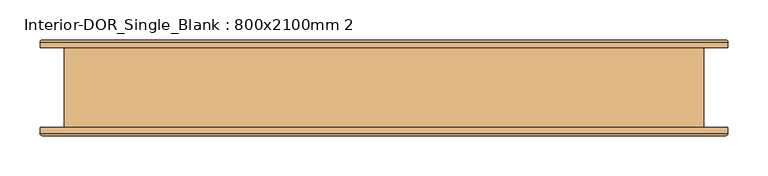
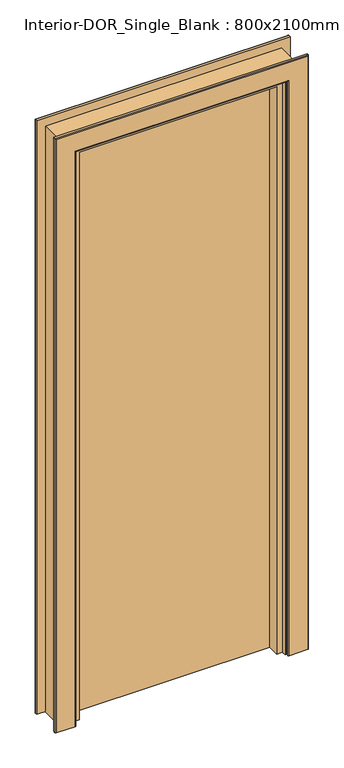
"""IFC4 building model written with IfcOpenShell, lengths in millimetres: door geometry, Interior-DOR_Single_Blank : 800x2100mm 2."""

import ifcopenshell
import ifcopenshell.guid

model = None  # the IFC model being written
_history = None  # IfcOwnerHistory: only IFC2X3 demands one
_inside = {}  # id of a spatial element -> (the spatial element, [elements in it])
_under = {}  # id of a project, library or spatial element -> (it, [spatial elements below it])
_declared = {}  # id of a project -> (the project, [libraries it declares])
_typed = {}  # id of a type object -> (the type object, [elements of that type])
_made_of = {}  # id of a material, layer set ... -> (it, [elements and type objects made of it])


def new_model(schema):
    """Start an empty IFC model of exactly this schema.

    Asked for "IFC4X3", IfcOpenShell would pick the latest addendum, in which some entities
    have other attributes; the version numbers below select the first issue.
    IFC2X3 requires an IfcOwnerHistory on every rooted entity: one is made here for all.
    """
    global model, _history
    if schema == "IFC4X3":
        model = ifcopenshell.file(schema_version=(4, 3, 0, 0))
    else:
        model = ifcopenshell.file(schema=schema)
    _inside.clear()
    _under.clear()
    _declared.clear()
    _typed.clear()
    _made_of.clear()
    _history = None
    if model.schema == "IFC2X3":
        org = make("IfcOrganization", Name="unknown")
        user = make(
            "IfcPersonAndOrganization",
            ThePerson=make("IfcPerson", FamilyName="unknown"),
            TheOrganization=org,
        )
        app = make(
            "IfcApplication",
            ApplicationDeveloper=org,
            Version="unknown",
            ApplicationFullName="unknown",
            ApplicationIdentifier="unknown",
        )
        _history = make(
            "IfcOwnerHistory",
            OwningUser=user,
            OwningApplication=app,
            ChangeAction="ADDED",
            CreationDate=0,
        )
    return model


def make(cls, **values):
    """One entity of the class cls with the attributes given. An attribute that is None is left unset."""
    return model.create_entity(
        cls, **{name: value for name, value in values.items() if value is not None}
    )


def rooted(cls, **values):
    """An entity with a GlobalId (a new one), such as an element, a storey or a relation."""
    return make(cls, GlobalId=ifcopenshell.guid.new(), OwnerHistory=_history, **values)


def si_unit(unit_type, name, prefix=None):
    """IfcSIUnit, for example si_unit("LENGTHUNIT", "METRE", prefix="MILLI")."""
    return make("IfcSIUnit", UnitType=unit_type, Prefix=prefix, Name=name)


def assignment(units):
    """IfcUnitAssignment: the units of a project."""
    return None if units is None else make("IfcUnitAssignment", Units=units)


def point(xyz):
    """IfcCartesianPoint."""
    return None if xyz is None else make("IfcCartesianPoint", Coordinates=xyz)


def direction(xyz):
    """IfcDirection."""
    return None if xyz is None else make("IfcDirection", DirectionRatios=xyz)


def frame(location, z_axis=None, x_axis=None):
    """IfcAxis2Placement3D, a coordinate frame: its origin and axes. An axis left out is left unset."""
    return make(
        "IfcAxis2Placement3D",
        Location=point(location),
        Axis=direction(z_axis),
        RefDirection=direction(x_axis),
    )


def origin():
    """The frame at (0, 0, 0) with its axes left unset."""
    return frame((0.0, 0.0, 0.0))


def origin_with_axes():
    """The frame at (0, 0, 0) with the z axis (0, 0, 1) and the x axis (1, 0, 0) written out."""
    return frame((0.0, 0.0, 0.0), z_axis=(0.0, 0.0, 1.0), x_axis=(1.0, 0.0, 0.0))


def place(relative_to, where):
    """IfcLocalPlacement: puts the frame where relative to a parent placement (None: the world)."""
    return make(
        "IfcLocalPlacement", PlacementRelTo=relative_to, RelativePlacement=where
    )


def context(
    kind, dimensions, precision=None, world=None, true_north=None, identifier=None
):
    """IfcGeometricRepresentationContext, for example the 3D "Model" context."""
    return make(
        "IfcGeometricRepresentationContext",
        ContextIdentifier=identifier,
        ContextType=kind,
        CoordinateSpaceDimension=dimensions,
        Precision=precision,
        WorldCoordinateSystem=world,
        TrueNorth=true_north,
    )


def project(units=None, contexts=None):
    """IfcProject with its units and contexts."""
    return rooted(
        "IfcProject",
        Name="project",
        RepresentationContexts=contexts,
        UnitsInContext=assignment(units),
    )


def spatial(cls, under=None, at=None, **own):
    """A site, building, storey or space (cls), placed at a placement, below another one or the project."""
    s = rooted(cls, ObjectPlacement=at, **own)
    if under is not None:
        _under.setdefault(under.id(), (under, []))[1].append(s)
    return s


def polyline(points):
    """IfcPolyline through the points."""
    return make("IfcPolyline", Points=[point(p) for p in points])


def circle_curve(where, radius):
    """IfcCircle in the frame where."""
    return make("IfcCircle", Position=where, Radius=radius)


def ellipse_curve(where, semi_axis1, semi_axis2):
    """IfcEllipse in the frame where."""
    return make(
        "IfcEllipse", Position=where, SemiAxis1=semi_axis1, SemiAxis2=semi_axis2
    )


def outline(outer, holes=None, kind="AREA"):
    """IfcArbitraryClosedProfileDef: a profile drawn as a closed curve; with holes, ...WithVoids."""
    if holes is None:
        return make("IfcArbitraryClosedProfileDef", ProfileType=kind, OuterCurve=outer)
    return make(
        "IfcArbitraryProfileDefWithVoids",
        ProfileType=kind,
        OuterCurve=outer,
        InnerCurves=holes,
    )


def extrude(swept, where, along, depth):
    """IfcExtrudedAreaSolid: the profile swept, set in the frame where, extruded along a direction by depth."""
    return make(
        "IfcExtrudedAreaSolid",
        SweptArea=swept,
        Position=where,
        ExtrudedDirection=direction(along),
        Depth=depth,
    )


def faces_of(points, faces, orient=None, outer=None):
    """IfcFace entities. A face is a list of loops; a loop is a list of indices into points, from 0.

    orient and outer hold one flag for each loop. By default every Orientation is true, the
    first loop of a face is its IfcFaceOuterBound and the others are IfcFaceBound.
    """
    made = []
    for i, loops in enumerate(faces):
        bounds = []
        for j, loop in enumerate(loops):
            is_outer = j == 0 if outer is None else outer[i][j]
            bounds.append(
                make(
                    "IfcFaceOuterBound" if is_outer else "IfcFaceBound",
                    Bound=make("IfcPolyLoop", Polygon=[points[k] for k in loop]),
                    Orientation=True if orient is None else orient[i][j],
                )
            )
        made.append(make("IfcFace", Bounds=bounds))
    return made


def faceted_brep(points, faces, orient=None, outer=None, voids=None):
    """IfcFacetedBrep: a solid bounded by flat faces; with voids (closed shells), ...WithVoids."""
    shared = [point(p) for p in points]
    hull = make("IfcClosedShell", CfsFaces=faces_of(shared, faces, orient, outer))
    if voids is None:
        return make("IfcFacetedBrep", Outer=hull)
    return make(
        "IfcFacetedBrepWithVoids",
        Outer=hull,
        Voids=[
            make(cls, CfsFaces=faces_of(shared, fs, o, b)) for cls, fs, o, b in voids
        ],
    )


def shape(context_of_items, identifier, shape_type, items):
    """IfcShapeRepresentation: the items that make up one representation, for example the "Body"."""
    return make(
        "IfcShapeRepresentation",
        ContextOfItems=context_of_items,
        RepresentationIdentifier=identifier,
        RepresentationType=shape_type,
        Items=items,
    )


def source(mapping_origin, context_of_items, identifier, shape_type, items):
    """IfcRepresentationMap: a shape defined once, which mapped items show again and again."""
    return make(
        "IfcRepresentationMap",
        MappingOrigin=mapping_origin,
        MappedRepresentation=shape(context_of_items, identifier, shape_type, items),
    )


def transform(
    local_origin,
    x_axis=None,
    y_axis=None,
    z_axis=None,
    scale=None,
    scale2=None,
    scale3=None,
    uniform=True,
):
    """IfcCartesianTransformationOperator3D, or its non-uniform kind. x_axis, y_axis, z_axis: its Axis1, 2, 3."""
    if uniform:
        return make(
            "IfcCartesianTransformationOperator3D",
            Axis1=direction(x_axis),
            Axis2=direction(y_axis),
            LocalOrigin=point(local_origin),
            Scale=scale,
            Axis3=direction(z_axis),
        )
    return make(
        "IfcCartesianTransformationOperator3DnonUniform",
        Axis1=direction(x_axis),
        Axis2=direction(y_axis),
        LocalOrigin=point(local_origin),
        Scale=scale,
        Axis3=direction(z_axis),
        Scale2=scale2,
        Scale3=scale3,
    )


def mapped(mapping_source, mapping_target):
    """IfcMappedItem: shows the shape of a source again, moved by a transform."""
    return make(
        "IfcMappedItem", MappingSource=mapping_source, MappingTarget=mapping_target
    )


def made_of(thing, what):
    """Note that an element or type object is made of a material, layer set ...; save() writes the relation."""
    if what is not None:
        _made_of.setdefault(what.id(), (what, []))[1].append(thing)
    return thing


def element(
    cls,
    number,
    at=None,
    inside=None,
    cuts=None,
    type_object=None,
    material=None,
    context=None,
    identifier="Body",
    shape_type=None,
    held_by="IfcProductDefinitionShape",
    body=None,
    shapes=None,
    **own,
):
    """One element of the class cls, such as IfcWall. Its Tag is "e" and its number.

    at: its placement. inside: the storey or other place that contains it. cuts: it is an
    opening in that element (IfcRelVoidsElement). A single representation is given by context,
    identifier, shape_type and body (its items); several are given by shapes. held_by: the class
    of the entity that holds the representations. save() writes the other relations.
    """
    e = rooted(cls, Tag="e%d" % number, ObjectPlacement=at, **own)
    if body is not None:
        shapes = [shape(context, identifier, shape_type, body)]
    if shapes is not None:
        e.Representation = make(held_by, Representations=shapes)
    if inside is not None:
        _inside.setdefault(inside.id(), (inside, []))[1].append(e)
    if cuts is not None:
        rooted(
            "IfcRelVoidsElement", RelatingBuildingElement=cuts, RelatedOpeningElement=e
        )
    if type_object is not None:
        _typed.setdefault(type_object.id(), (type_object, []))[1].append(e)
    return made_of(e, material)


def aggregate(whole, parts):
    """IfcRelAggregates: a whole, such as a stair, and the parts it consists of."""
    return rooted("IfcRelAggregates", RelatingObject=whole, RelatedObjects=parts)


def save(model, path):
    """Write the relations noted so far, then the file.

    IfcRelAggregates (storeys below a building ...), IfcRelContainedInSpatialStructure (elements
    in a storey), IfcRelDefinesByType, IfcRelAssociatesMaterial and IfcRelDeclares: one each for
    every whole, place, type object, material and project.
    """
    for whole, parts in _under.values():
        aggregate(whole, parts)
    for where, things in _inside.values():
        rooted(
            "IfcRelContainedInSpatialStructure",
            RelatedElements=things,
            RelatingStructure=where,
        )
    for kind, things in _typed.values():
        rooted("IfcRelDefinesByType", RelatedObjects=things, RelatingType=kind)
    for what, things in _made_of.values():
        rooted("IfcRelAssociatesMaterial", RelatedObjects=things, RelatingMaterial=what)
    for by, libraries in _declared.values():
        rooted("IfcRelDeclares", RelatingContext=by, RelatedDefinitions=libraries)
    model.write(path)


def plane_surface(at):
    """IfcPlane: the flat surface through the origin of the frame at, square to its z axis."""
    return make("IfcPlane", Position=at)


def cylinder_surface(at, radius):
    """IfcCylindricalSurface: all points at the distance radius from the z axis of the frame at."""
    return make("IfcCylindricalSurface", Position=at, Radius=radius)


def advanced_brep(points, edges, surfaces, faces):
    """IfcAdvancedBrep: a solid bounded by faces that lie on surfaces and meet in shared edges.

    An edge is (start, end): straight between two places in points (the first is 0);
    or (start, end, curve); or (start, end, curve, False) where it runs against its curve.
    A face is (place in surfaces, loops), or (place, loops, False) where it looks against
    its surface's normal. A loop lists edges by number (the first is 1), with a minus sign
    where the edge is run from its end to its start. The first loop is the outer one.
    """
    corners = [point(p) for p in points]
    vertices = [make("IfcVertexPoint", VertexGeometry=c) for c in corners]
    made = []
    for start, end, *more in edges:
        made.append(
            make(
                "IfcEdgeCurve",
                EdgeStart=vertices[start],
                EdgeEnd=vertices[end],
                EdgeGeometry=more[0] if more else make("IfcPolyline", Points=[corners[start], corners[end]]),
                SameSense=more[1] if len(more) > 1 else True,
            )
        )
    hull = []
    for where, loops, *sense in faces:
        bounds = []
        for j, loop in enumerate(loops):
            ring = [make("IfcOrientedEdge", EdgeElement=made[abs(k) - 1], Orientation=k > 0) for k in loop]
            bounds.append(
                make(
                    "IfcFaceOuterBound" if j == 0 else "IfcFaceBound",
                    Bound=make("IfcEdgeLoop", EdgeList=ring),
                    Orientation=True,
                )
            )
        hull.append(make("IfcAdvancedFace", Bounds=bounds, FaceSurface=surfaces[where], SameSense=sense[0] if sense else True))
    return make("IfcAdvancedBrep", Outer=make("IfcClosedShell", CfsFaces=hull))


def interior_dor_single_blank_800x2100mm_2_9dcdbc73(model_context):
    return source(origin(), model_context, "Body", "SolidModel", [
        advanced_brep(
        [(-360.0, 50.0, 0.0), (-430.0, 50.0, 0.0), (-430.0, 57.0, 0.0), (-427.0, 60.0, 0.0), (-363.0, 60.0, 0.0), (-360.0, 57.0, 0.0), (-360.0, 57.0, 2060.0), (-360.0, 50.0, 2060.0), (-363.0, 60.0, 2063.0), (-427.0, 60.0, 2127.0), (427.0, 60.0, 2127.0), (427.0, 60.0, 0.0), (363.0, 60.0, 0.0), (363.0, 60.0, 2063.0), (-430.0, 57.0, 2130.0), (-430.0, 50.0, 2130.0), (360.0, 50.0, 2060.0), (360.0, 50.0, 0.0), (430.0, 50.0, 0.0), (430.0, 50.0, 2130.0), (360.0, 57.0, 0.0), (360.0, 57.0, 2060.0), (430.0, 57.0, 0.0), (430.0, 57.0, 2130.0)],
        [
            (0, 1),
            (1, 2),
            (2, 3, circle_curve(frame((-427.0, 57.0, 0.0), z_axis=(0.0, 0.0, -1.0), x_axis=(-1.0, 0.0, 0.0)), 3.0)),
            (3, 4),
            (4, 5, circle_curve(frame((-363.0, 57.0, 0.0), z_axis=(0.0, 0.0, -1.0), x_axis=(-1.0, 0.0, 0.0)), 3.0)),
            (5, 0),
            (5, 6),
            (6, 7),
            (7, 0),
            (4, 8),
            (8, 6, ellipse_curve(frame((-363.0, 57.0, 2063.0), z_axis=(-0.7071067811865475, 0.0, -0.7071067811865475), x_axis=(0.7071067811865474, 0.0, -0.7071067811865476)), 4.2426407, 3.0)),
            (3, 9),
            (9, 10),
            (10, 11),
            (11, 12),
            (12, 13),
            (13, 8),
            (2, 14),
            (14, 9, ellipse_curve(frame((-427.0, 57.0, 2127.0), z_axis=(-0.7071067811865475, 0.0, -0.7071067811865475), x_axis=(0.7071067811865474, 0.0, -0.7071067811865476)), 4.2426407, 3.0)),
            (1, 15),
            (15, 14),
            (7, 16),
            (16, 17),
            (17, 18),
            (18, 19),
            (19, 15),
            (12, 20, circle_curve(frame((363.0, 57.0, 0.0), z_axis=(0.0, 0.0, 1.0), x_axis=(1.0, 0.0, 0.0)), 3.0)),
            (20, 21),
            (21, 13, ellipse_curve(frame((363.0, 57.0, 2063.0), z_axis=(0.7071067811865475, 0.0, -0.7071067811865475), x_axis=(0.7071067811865474, 0.0, 0.7071067811865476)), 4.2426407, 3.0)),
            (17, 20),
            (11, 22, circle_curve(frame((427.0, 57.0, 0.0), z_axis=(0.0, 0.0, -1.0), x_axis=(1.0, 0.0, 0.0)), 3.0)),
            (22, 18),
            (23, 22),
            (10, 23, ellipse_curve(frame((427.0, 57.0, 2127.0), z_axis=(0.7071067811865475, 0.0, -0.7071067811865475), x_axis=(0.7071067811865474, 0.0, 0.7071067811865476)), 4.2426407, 3.0)),
            (23, 19),
            (16, 21),
            (6, 21),
            (14, 23),
        ],
        [
            plane_surface(frame((-400.0, -50.0, 0.0), z_axis=(0.0, 0.0, -1.0), x_axis=(0.0, 1.0, 0.0))),
            plane_surface(frame((-360.0, 50.0, 0.0), z_axis=(1.0, 0.0, 0.0), x_axis=(0.0, 0.0, 1.0))),
            cylinder_surface(frame((-363.0, 57.0, 0.0), z_axis=(0.0, 0.0, -1.0), x_axis=(-1.0, 0.0, 0.0)), 3.0),
            plane_surface(frame((-363.0, 60.0, 0.0), z_axis=(0.0, 1.0, 0.0), x_axis=(0.0, 0.0, 1.0))),
            cylinder_surface(frame((-427.0, 57.0, 0.0), z_axis=(0.0, 0.0, -1.0), x_axis=(-1.0, 0.0, 0.0)), 3.0),
            plane_surface(frame((-430.0, 57.0, 0.0), z_axis=(-1.0, 0.0, 0.0), x_axis=(0.0, 0.0, 1.0))),
            plane_surface(frame((-430.0, 50.0, 0.0), z_axis=(0.0, -1.0, 0.0), x_axis=(0.0, 0.0, 1.0))),
            cylinder_surface(frame((363.0, 57.0, 2100.0), z_axis=(0.0, 0.0, 1.0), x_axis=(1.0, 0.0, 0.0)), 3.0),
            plane_surface(frame((400.0, -50.0, 0.0), z_axis=(0.0, 0.0, -1.0), x_axis=(0.0, 1.0, 0.0))),
            cylinder_surface(frame((427.0, 57.0, 2100.0), z_axis=(0.0, 0.0, 1.0), x_axis=(1.0, 0.0, 0.0)), 3.0),
            plane_surface(frame((430.0, 57.0, 2130.0), z_axis=(1.0, 0.0, 0.0), x_axis=(0.0, 0.0, -1.0))),
            plane_surface(frame((360.0, 50.0, 2060.0), z_axis=(-1.0, 0.0, 0.0), x_axis=(0.0, 0.0, -1.0))),
            plane_surface(frame((-360.0, 50.0, 2060.0), z_axis=(0.0, 0.0, -1.0), x_axis=(1.0, 0.0, 0.0))),
            cylinder_surface(frame((-400.0, 57.0, 2063.0), z_axis=(-1.0, 0.0, 0.0), x_axis=(0.0, 0.0, 1.0)), 3.0),
            cylinder_surface(frame((-400.0, 57.0, 2127.0), z_axis=(-1.0, 0.0, 0.0), x_axis=(0.0, 0.0, 1.0)), 3.0),
            plane_surface(frame((-430.0, 57.0, 2130.0), z_axis=(0.0, 0.0, 1.0), x_axis=(1.0, 0.0, 0.0))),
        ],
        [
            (0, [[1, 2, 3, 4, 5, 6]]),
            (1, [[7, 8, 9, -6]]),
            (2, [[10, 11, -7, -5]]),
            (3, [[12, 13, 14, 15, 16, 17, -10, -4]]),
            (4, [[18, 19, -12, -3]]),
            (5, [[20, 21, -18, -2]]),
            (6, [[-9, 22, 23, 24, 25, 26, -20, -1]]),
            (7, [[-16, 27, 28, 29]]),
            (8, [[30, -27, -15, 31, 32, -24]]),
            (9, [[33, -31, -14, 34]]),
            (10, [[-25, -32, -33, 35]]),
            (11, [[-28, -30, -23, 36]]),
            (12, [[37, -36, -22, -8]]),
            (13, [[-17, -29, -37, -11]]),
            (14, [[38, -34, -13, -19]]),
            (15, [[-26, -35, -38, -21]]),
        ],
    ),
        advanced_brep(
        [(-430.0, -50.0, 0.0), (-360.0, -50.0, 0.0), (-360.0, -57.0, 0.0), (-363.0, -60.0, 0.0), (-427.0, -60.0, 0.0), (-430.0, -57.0, 0.0), (-430.0, -57.0, 2130.0), (-430.0, -50.0, 2130.0), (-427.0, -60.0, 2127.0), (-363.0, -60.0, 2063.0), (363.0, -60.0, 2063.0), (363.0, -60.0, 0.0), (427.0, -60.0, 0.0), (427.0, -60.0, 2127.0), (-360.0, -57.0, 2060.0), (-360.0, -50.0, 2060.0), (430.0, -50.0, 2130.0), (430.0, -50.0, 0.0), (360.0, -50.0, 0.0), (360.0, -50.0, 2060.0), (430.0, -57.0, 0.0), (430.0, -57.0, 2130.0), (360.0, -57.0, 0.0), (360.0, -57.0, 2060.0)],
        [
            (0, 1),
            (1, 2),
            (2, 3, circle_curve(frame((-363.0, -57.0, 0.0), z_axis=(0.0, 0.0, -1.0), x_axis=(-1.0, 0.0, 0.0)), 3.0)),
            (3, 4),
            (4, 5, circle_curve(frame((-427.0, -57.0, 0.0), z_axis=(0.0, 0.0, -1.0), x_axis=(-1.0, 0.0, 0.0)), 3.0)),
            (5, 0),
            (5, 6),
            (6, 7),
            (7, 0),
            (4, 8),
            (8, 6, ellipse_curve(frame((-427.0, -57.0, 2127.0), z_axis=(-0.7071067811865475, 0.0, -0.7071067811865475), x_axis=(0.7071067811865474, 0.0, -0.7071067811865476)), 4.2426407, 3.0)),
            (3, 9),
            (9, 10),
            (10, 11),
            (11, 12),
            (12, 13),
            (13, 8),
            (2, 14),
            (14, 9, ellipse_curve(frame((-363.0, -57.0, 2063.0), z_axis=(-0.7071067811865475, 0.0, -0.7071067811865475), x_axis=(0.7071067811865474, 0.0, -0.7071067811865476)), 4.2426407, 3.0)),
            (1, 15),
            (15, 14),
            (7, 16),
            (16, 17),
            (17, 18),
            (18, 19),
            (19, 15),
            (12, 20, circle_curve(frame((427.0, -57.0, 0.0), z_axis=(0.0, 0.0, 1.0), x_axis=(1.0, 0.0, 0.0)), 3.0)),
            (20, 21),
            (21, 13, ellipse_curve(frame((427.0, -57.0, 2127.0), z_axis=(0.7071067811865475, 0.0, -0.7071067811865475), x_axis=(0.7071067811865474, 0.0, 0.7071067811865476)), 4.2426407, 3.0)),
            (17, 20),
            (11, 22, circle_curve(frame((363.0, -57.0, 0.0), z_axis=(0.0, 0.0, -1.0), x_axis=(1.0, 0.0, 0.0)), 3.0)),
            (22, 18),
            (23, 22),
            (10, 23, ellipse_curve(frame((363.0, -57.0, 2063.0), z_axis=(0.7071067811865475, 0.0, -0.7071067811865475), x_axis=(0.7071067811865474, 0.0, 0.7071067811865476)), 4.2426407, 3.0)),
            (23, 19),
            (16, 21),
            (6, 21),
            (14, 23),
        ],
        [
            plane_surface(frame((-400.0, -50.0, 0.0), z_axis=(0.0, 0.0, -1.0), x_axis=(0.0, 1.0, 0.0))),
            plane_surface(frame((-430.0, -50.0, 0.0), z_axis=(-1.0, 0.0, 0.0), x_axis=(0.0, 0.0, 1.0))),
            cylinder_surface(frame((-427.0, -57.0, 0.0), z_axis=(0.0, 0.0, -1.0), x_axis=(-1.0, 0.0, 0.0)), 3.0),
            plane_surface(frame((-427.0, -60.0, 0.0), z_axis=(0.0, -1.0, 0.0), x_axis=(0.0, 0.0, 1.0))),
            cylinder_surface(frame((-363.0, -57.0, 0.0), z_axis=(0.0, 0.0, -1.0), x_axis=(-1.0, 0.0, 0.0)), 3.0),
            plane_surface(frame((-360.0, -57.0, 0.0), z_axis=(1.0, 0.0, 0.0), x_axis=(0.0, 0.0, 1.0))),
            plane_surface(frame((-360.0, -50.0, 0.0), z_axis=(0.0, 1.0, 0.0), x_axis=(0.0, 0.0, 1.0))),
            cylinder_surface(frame((427.0, -57.0, 2100.0), z_axis=(0.0, 0.0, 1.0), x_axis=(1.0, 0.0, 0.0)), 3.0),
            plane_surface(frame((400.0, -50.0, 0.0), z_axis=(0.0, 0.0, -1.0), x_axis=(0.0, 1.0, 0.0))),
            cylinder_surface(frame((363.0, -57.0, 2100.0), z_axis=(0.0, 0.0, 1.0), x_axis=(1.0, 0.0, 0.0)), 3.0),
            plane_surface(frame((360.0, -57.0, 2060.0), z_axis=(-1.0, 0.0, 0.0), x_axis=(0.0, 0.0, -1.0))),
            plane_surface(frame((430.0, -50.0, 2130.0), z_axis=(1.0, 0.0, 0.0), x_axis=(0.0, 0.0, -1.0))),
            plane_surface(frame((-430.0, -50.0, 2130.0), z_axis=(0.0, 0.0, 1.0), x_axis=(1.0, 0.0, 0.0))),
            cylinder_surface(frame((-400.0, -57.0, 2127.0), z_axis=(-1.0, 0.0, 0.0), x_axis=(0.0, 0.0, 1.0)), 3.0),
            cylinder_surface(frame((-400.0, -57.0, 2063.0), z_axis=(-1.0, 0.0, 0.0), x_axis=(0.0, 0.0, 1.0)), 3.0),
            plane_surface(frame((-360.0, -57.0, 2060.0), z_axis=(0.0, 0.0, -1.0), x_axis=(1.0, 0.0, 0.0))),
        ],
        [
            (0, [[1, 2, 3, 4, 5, 6]]),
            (1, [[7, 8, 9, -6]]),
            (2, [[10, 11, -7, -5]]),
            (3, [[12, 13, 14, 15, 16, 17, -10, -4]]),
            (4, [[18, 19, -12, -3]]),
            (5, [[20, 21, -18, -2]]),
            (6, [[-9, 22, 23, 24, 25, 26, -20, -1]]),
            (7, [[-16, 27, 28, 29]]),
            (8, [[30, -27, -15, 31, 32, -24]]),
            (9, [[33, -31, -14, 34]]),
            (10, [[-25, -32, -33, 35]]),
            (11, [[-28, -30, -23, 36]]),
            (12, [[37, -36, -22, -8]]),
            (13, [[-17, -29, -37, -11]]),
            (14, [[38, -34, -13, -19]]),
            (15, [[-26, -35, -38, -21]]),
        ],
    ),
        faceted_brep([(-400.0, -50.0, 0.0), (-400.0, 50.0, 0.0), (-355.0, 50.0, 0.0), (-355.0, 5.0, 0.0), (-335.0, 5.0, 0.0), (-335.0, -35.0, 0.0), (-355.0, -35.0, 0.0), (-355.0, -50.0, 0.0), (-355.0, -50.0, 2055.0), (355.0, -50.0, 2055.0), (355.0, -50.0, 0.0), (400.0, -50.0, 0.0), (400.0, -50.0, 2100.0), (-400.0, -50.0, 2100.0), (-355.0, -35.0, 2055.0), (-335.0, -35.0, 2035.0), (335.0, -35.0, 2035.0), (335.0, -35.0, 0.0), (355.0, -35.0, 0.0), (355.0, -35.0, 2055.0), (-335.0, 5.0, 2035.0), (-355.0, 5.0, 2055.0), (355.0, 5.0, 2055.0), (355.0, 5.0, 0.0), (335.0, 5.0, 0.0), (335.0, 5.0, 2035.0), (-355.0, 50.0, 2055.0), (-400.0, 50.0, 2100.0), (400.0, 50.0, 2100.0), (400.0, 50.0, 0.0), (355.0, 50.0, 0.0), (355.0, 50.0, 2055.0)], [[[0, 1, 2, 3, 4, 5, 6, 7]], [[7, 8, 9, 10, 11, 12, 13, 0]], [[6, 14, 8, 7]], [[5, 15, 16, 17, 18, 19, 14, 6]], [[4, 20, 15, 5]], [[3, 21, 22, 23, 24, 25, 20, 4]], [[2, 26, 21, 3]], [[1, 27, 28, 29, 30, 31, 26, 2]], [[0, 13, 27, 1]], [[12, 11, 29, 28]], [[11, 10, 18, 17, 24, 23, 30, 29]], [[19, 18, 10, 9]], [[25, 24, 17, 16]], [[31, 30, 23, 22]], [[20, 25, 16, 15]], [[26, 31, 22, 21]], [[13, 12, 28, 27]], [[14, 19, 9, 8]]]),
        extrude(outline(polyline([(355.0, 50.0), (355.0, 5.0), (-355.0, 5.0), (-355.0, 50.0), (355.0, 50.0)])), origin_with_axes(), (0.0, 0.0, 1.0), 2055.0),
    ])


if __name__ == "__main__":
    model = new_model("IFC4")
    model_context = context("Model", 3, world=origin())
    ifc_project = project(units=[si_unit("LENGTHUNIT", "METRE", prefix="MILLI")], contexts=[model_context])
    site = spatial("IfcSite", under=ifc_project)
    building = spatial("IfcBuilding", under=site)
    placement = place(None, origin())
    interior_dor_single_blank_800x2100mm_2_shape = interior_dor_single_blank_800x2100mm_2_9dcdbc73(model_context)
    element("IfcDoor", 1, ObjectType="Interior-DOR_Single_Blank : 800x2100mm 2", at=placement, inside=building, context=model_context, shape_type="MappedRepresentation", body=[
        mapped(interior_dor_single_blank_800x2100mm_2_shape, transform((0.0, 0.0, 0.0), x_axis=(1.0, 0.0, 0.0), y_axis=(0.0, 1.0, 0.0), z_axis=(0.0, 0.0, 1.0))),
    ])
    save(model, "model.ifc")

# Revit data of these elements
# Type "Interior-DOR_Single_Blank : 800x2100mm 2"
#   Type IfcGUID = "0dwJ1JWsv3L8A_XhzwP5MW"
#   Assembly Code = "C1020120"
#   Type Mark = "195"
#   Classification.Uniclass.EF.Number = "EF_25_30"
#   Classification.Uniclass.EF.Description = "Doors and windows"
#   WindLoadRating = "n/a"
#   WaterTightnessRating = "n/a"
#   WarrantyStartDate [instance default] = "1900-12-31T23:59:59"
#   WarrantyGuarantorParts = "n/a"
#   WarrantyGuarantorLabor = "n/a"
#   WarrantyDurationUnit = "year"
#   WarrantyDurationParts = "n/a"
#   WarrantyDurationLabor = "n/a"
#   WarrantyDescription = "n/a"
#   Version = "2"
#   Uniclass2015Version = "Systems v1.9"
#   Uniclass2015Title = "Doorset systems"
#   Uniclass2015Code = "Ss_25_30_20_25"
#   URL = "www.nationalbimlibrary.com"
#   TagNumber [instance default] = "n/a"
#   SustainabilityPerformance = "n/a"
#   Status = "UNSET"
#   Size = "1010 x 2100 mm"
#   Shape = "n/a"
#   SerialNumber [instance default] = "n/a"
#   SecurityRating = "n/a"
#   Revision = "n/a"
#   ReplacementCost = "n/a"
#   Reference = "n/a"
#   ProductInformation = "n/a"
#   Operation = "SINGLE_SWING_RIGHT"
#   OmniClassVersion = "Table 22 2012-05-16"
#   OmniClassTitle = "Doors and Frames"
#   OmniClassCode = "22-08 10 00"
#   Name = "DoorsetSystem_Interior-Single_Blank"
#   NBSReference = "25-50-20/120"
#   NBSDescription = "Doorset system"
#   NBSCertification = "www.nationalbimlibrary.com/cert/mlf45nxc"
#   ModelReference = "Interior Single Door"
#   ModelNumber = "n/a"
#   Model = "Interior Single Door"
#   MechanicalLoadRating = "n/a"
#   Material = "n/a"
#   ManufacturerURL = "n/a"
#   ManufacturerName = "n/a"
#   Manufacturer = "info@theNBS.com"
#   InstallationDate [instance default] = "1900-12-31T23:59:59"
#   IfcExportType = "DOOR"
#   IfcExportAs = "IfcDoorType"
#   HygrothermalRating = "n/a"
#   Grade = "n/a"
#   FireRating = "n/a"
#   Fire Rating = "n/a"
#   Finish = "n/a"
#   Features = "n/a"
#   ExpectedLife = "n/a"
#   DurationUnit = "n/a"
#   DurabilityRating = "n/a"
#   DoorNumber [instance default] = "n/a"
#   Description = "Generic single interior door"
#   Construction Type = "USERDEFINED"
#   Constituents = "n/a"
#   ComponentNumber [instance default] = "n/a"
#   Color = "n/a"
#   CodePerformance = "n/a"
#   Category = "Ss_25_30_20_25:Doorset systems"
#   BarCode [instance default] = "n/a"
#   BIMObjectName = "NBS_DoorsetSystem_Interior-Single_Blank"
#   Author = "NBS"
#   AssetType = "Fixed"
#   AssetIdentifier [instance default] = "n/a"
#   AcousticRating = "n/a"
#   AccessibilityPerformance = "n/a"
#   Width = 0.8 m
#   WallThickness [instance default] = 0.15 m
#   ThresholdHeight = 0.015 m
#   Thickness = 0.15 m
#   ThermalTransmittance = 0
#   StructuralToleranceJamb = 0 m
#   StructuralToleranceHead = 0 m
#   StructuralOpeningWidth = 0.8 m
#   StructuralOpeningHeight = 2.1 m
#   StopProjection = 0.02 m
#   StopDepth = 0.04 m
#   Rough Width [instance default] = 0.8 m
#   Rough Height [instance default] = 2.1 m
#   RebateDepth = 0.045 m
#   PanelWidth = 0.71 m
#   PanelUndercut = 0 m
#   PanelHeight = 2.055 m
#   PanelDepth = 0.045 m
#   OpeningTolerance = 0 m
#   NominalWidth = 0.8 m
#   NominalLength = 0 m
#   NominalHeight = 2.1 m
#   Infiltration = 0
#   Height = 2.1 m
#   GlazingAreaFraction = 0
#   FrameThickness = 0.045 m
#   FrameSetback [instance default] = 0 m
#   FrameDepth [instance default] = 0.15 m
#   FinishThicknessInternal [instance default] = 0 m
#   FinishThicknessExternal [instance default] = 0 m
#   ClearOpeningWidth = 0.67 m
#   ClearOpeningHeight = 2.035 m
#   CalculatedInteriorVoidDepth [instance default] = 0.3 m
#   ArchitraveWidth = 0.07 m
#   ArchitraveThickness = 0.01 m
#   ArchitraveSetbackFromFrameFace = 0.005 m
#   SmokeStop = no
#   SingleRebate = no
#   SelfClosing = no
#   PlantedStop = yes
#   IsExternal = no
#   HasDrive = no
#   HandicapAccessible = no
#   Wall Closure = 4
#   FireExit = no
#   ArchitraveFrontRequired [instance default] = yes
#   ArchitraveBackRequired [instance default] = yes
#   PanelMaterial = NBS_Concept
#   HardwareFinish = NBS_Concept
#   FrameSectionMaterial = NBS_Concept
#   Function = (empty or 0)
#   Cost = 0
# Element 1 (IfcDoor, "Interior-DOR_Single_Blank : 800x2100mm 2")
#   WallThickness = 0.1 m
#   FrameDepth = 0.1 m
#   Materials on its faces: "NBS_Concept"
# Materials
#   "NBS_Concept": class "Generic", colour RGB 255 255 255, transparency 0, Description = "To be specified", Cost = 0
